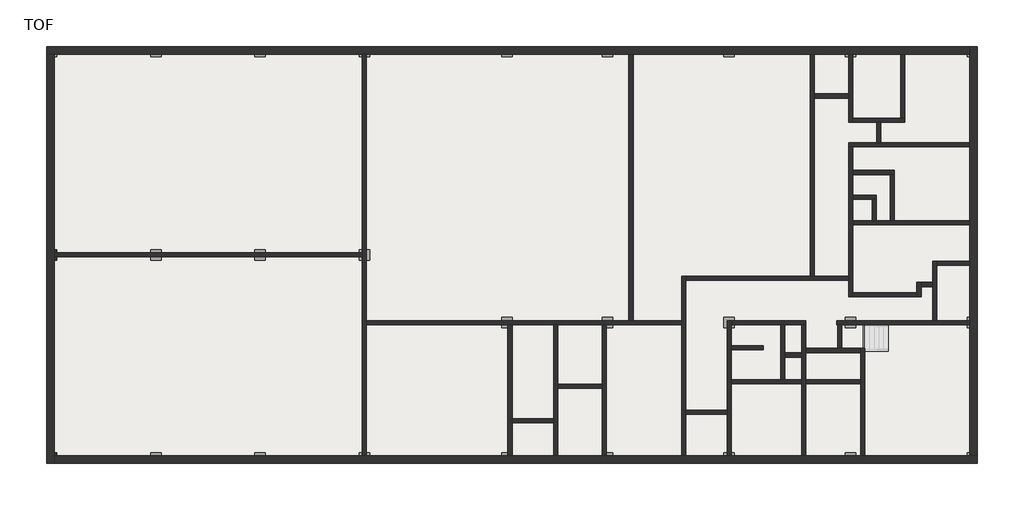
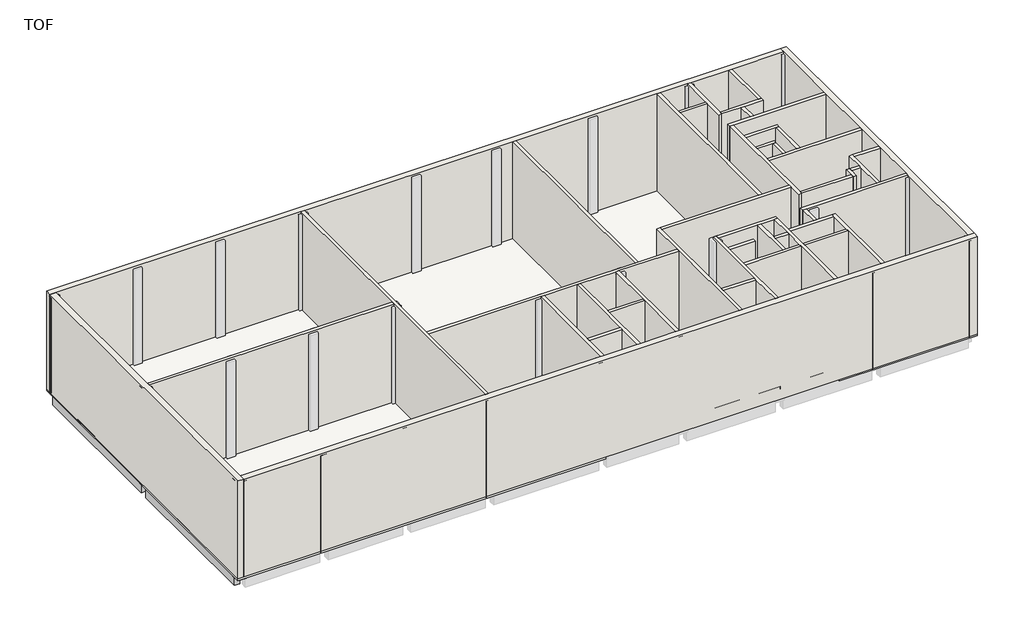
# One storey, part 1 of 2: 45 walls, 6 slabs, 2 beams, 2 columns.
# Revit data of these elements (continued)
# Element 13 (IfcWall, "H_WA_AMW_Brick Wall_Ext (0.5B_50_1.0B / Emulsion)") (continued)
#   Materials on its faces: "Default Wall"
# Element 14 (IfcWall, "H_WA_AMW_Brick Wall_Ext (0.5B_50_1.0B / Emulsion)")
#   Mark = "EW4"
#   Wall Loca = "EXT"
#   Wall Style Name = "Concrete Wall+Insulation+Gypsum Board"
#   Wall Base Material-2 = "Glass Wool (Fiberglass)"
#   Wall Base Material-3 = "Concrete Wall"
#   Wall Finish-Ex = "Acrylic Emulsion Paint on Fair Faced Concrete"
#   Top Offset = 0.000 mm
#   Base Offset = 0.000 mm
#   wall height = 7500.000 mm
#   Wall Style No = EW51-1
#   Phase Created = New Construction
#   Base Constraint = TOF
#   Top Constraint = TOC
#   Materials on its faces: "Default Wall"
# Element 15 (IfcWall, "H_WA_AMW_Block Wall_Int_T200 (Both Plaster_Emulsion)")
#   Mark = "W1"
#   Wall Loca = "INT"
#   Wall Style Name = "Block Wall"
#   Wall Ref. = ""
#   Wall Base Material-1 = "Concrete Block"
#   Wall Base Material-2 = ""
#   Wall Base Material-3 = ""
#   Wall Finish-Ex = ""
#   Top Offset = 0.000 mm
#   Base Offset = 0.000 mm
#   wall height = 7500.000 mm
#   Wall Style No = IW21
#   Phase Created = New Construction
#   Base Constraint = TOF
#   Top Constraint = TOC
#   Materials on its faces: "Default Wall"
# Element 16 (IfcWall, "H_WA_AMW_Block Wall_Int_T200 (Both Plaster_Emulsion)")
#   Mark = "W2"
#   Wall Loca = "INT"
#   Wall Style Name = "Block Wall"
#   Wall Ref. = ""
#   Wall Base Material-1 = "Concrete Block"
#   Wall Base Material-2 = ""
#   Wall Base Material-3 = ""
#   Wall Finish-Ex = ""
#   Top Offset = 0.000 mm
#   Base Offset = 0.000 mm
#   wall height = 7500.000 mm
#   Wall Style No = IW21
#   Phase Created = New Construction
#   Base Constraint = TOF
#   Top Constraint = TOC
#   Materials on its faces: "Default Wall"
# Element 17 (IfcWall, "H_WA_AMW_Block Wall_Int_T200 (Both Plaster_Emulsion)")
#   Mark = "W3"
#   Wall Loca = "INT"
#   Wall Style Name = "Block Wall"
#   Wall Ref. = ""
#   Wall Base Material-1 = "Concrete Block"
#   Wall Base Material-2 = ""
#   Wall Base Material-3 = ""
#   Wall Finish-Ex = ""
#   Top Offset = 0.000 mm
#   Base Offset = 0.000 mm
#   wall height = 7500.000 mm
#   Wall Style No = IW21
#   Phase Created = New Construction
#   Base Constraint = TOF
#   Top Constraint = TOC
#   Materials on its faces: "Default Wall"
# Element 18 (IfcWall, "H_WA_AMW_Block Wall_Int_T200 (Both Plaster_Emulsion)")
#   Mark = "W4"
#   Wall Loca = "INT"
#   Wall Style Name = "Block Wall"
#   Wall Ref. = ""
#   Wall Base Material-1 = "Concrete Block"
#   Wall Base Material-2 = ""
#   Wall Base Material-3 = ""
#   Wall Finish-Ex = ""
#   Top Offset = 0.000 mm
#   Base Offset = 0.000 mm
#   wall height = 7500.000 mm
#   Wall Style No = IW21
#   Phase Created = New Construction
#   Base Constraint = TOF
#   Top Constraint = TOC
#   Materials on its faces: "Default Wall"
# Element 19 (IfcWall, "H_WA_AMW_Block Wall_Int_T200 (Both Plaster_Emulsion)")
#   Mark = "W5"
#   Wall Loca = "INT"
#   Wall Style Name = "Block Wall"
#   Wall Ref. = ""
#   Wall Base Material-1 = "Concrete Block"
#   Wall Base Material-2 = ""
#   Wall Base Material-3 = ""
#   Wall Finish-Ex = ""
#   built-in parameter 1001111 = 1000.000 mm
#   Top Offset = 0.000 mm
#   Base Offset = 1000.000 mm
#   wall height = 6500.000 mm
#   Wall Style No = IW21
#   Phase Created = New Construction
#   Base Constraint = TOF
#   Top Constraint = TOC
#   Materials on its faces: "Default Wall"
# Element 20 (IfcWall, "H_WA_AMW_Block Wall_Int_T200 (Both Plaster_Emulsion)")
#   Mark = "W6"
#   Wall Loca = "INT"
#   Wall Style Name = "Block Wall"
#   Wall Ref. = ""
#   Wall Base Material-1 = "Concrete Block"
#   Wall Base Material-2 = ""
#   Wall Base Material-3 = ""
#   Wall Finish-Ex = ""
#   Top Offset = 0.000 mm
#   Base Offset = 0.000 mm
#   wall height = 7500.000 mm
#   Wall Style No = IW21
#   Phase Created = New Construction
#   Base Constraint = TOF
#   Top Constraint = TOC
#   Materials on its faces: "Default Wall"
# Element 21 (IfcWall, "H_WA_AMW_Block Wall_Int_T200 (Both Plaster_Emulsion)")
#   Mark = "W7"
#   Wall Loca = "INT"
#   Wall Style Name = "Block Wall"
#   Wall Ref. = ""
#   Wall Base Material-1 = "Concrete Block"
#   Wall Base Material-2 = ""
#   Wall Base Material-3 = ""
#   Wall Finish-Ex = ""
#   Top Offset = 0.000 mm
#   Base Offset = 0.000 mm
#   wall height = 7500.000 mm
#   Wall Style No = IW21
#   Phase Created = New Construction
#   Base Constraint = TOF
#   Top Constraint = TOC
#   Materials on its faces: "Default Wall"
# Element 22 (IfcWall, "H_WA_AMW_Block Wall_Int_T200 (Both Plaster_Emulsion)")
#   Mark = "W8"
#   Wall Loca = "INT"
#   Wall Style Name = "Block Wall"
#   Wall Ref. = ""
#   Wall Base Material-1 = "Concrete Block"
#   Wall Base Material-2 = ""
#   Wall Base Material-3 = ""
#   Wall Finish-Ex = ""
#   built-in parameter 1001111 = 1000.000 mm
#   Top Offset = 0.000 mm
#   Base Offset = 1000.000 mm
#   wall height = 6500.000 mm
#   Wall Style No = IW21
#   Phase Created = New Construction
#   Base Constraint = TOF
#   Top Constraint = TOC
#   Materials on its faces: "Default Wall"
# Element 23 (IfcWall, "H_WA_AMW_Block Wall_Int_T200 (Both Plaster_Emulsion)")
#   Mark = "W9"
#   Wall Loca = "INT"
#   Wall Style Name = "Block Wall"
#   Wall Ref. = ""
#   Wall Base Material-1 = "Concrete Block"
#   Wall Base Material-2 = ""
#   Wall Base Material-3 = ""
#   Wall Finish-Ex = ""
#   built-in parameter 1001111 = 1000.000 mm
#   Top Offset = 0.000 mm
#   Base Offset = 1000.000 mm
#   wall height = 6500.000 mm
#   Wall Style No = IW21
#   Phase Created = New Construction
#   Base Constraint = TOF
#   Top Constraint = TOC
#   Materials on its faces: "Default Wall"
# Element 24 (IfcWall, "H_WA_AMW_Block Wall_Int_T200 (Both Plaster_Emulsion)")
#   Mark = "W10"
#   Wall Loca = "INT"
#   Wall Style Name = "Block Wall"
#   Wall Ref. = ""
#   Wall Base Material-1 = "Concrete Block"
#   Wall Base Material-2 = ""
#   Wall Base Material-3 = ""
#   Wall Finish-Ex = ""
#   built-in parameter 1001111 = 1000.000 mm
#   Top Offset = 0.000 mm
#   Base Offset = 1000.000 mm
#   wall height = 6500.000 mm
#   Wall Style No = IW21
#   Phase Created = New Construction
#   Base Constraint = TOF
#   Top Constraint = TOC
#   Materials on its faces: "Default Wall"
# Element 25 (IfcWall, "H_WA_AMW_Block Wall_Int_T200 (Both Plaster_Emulsion)")
#   Mark = "W11"
#   Wall Loca = "INT"
#   Wall Style Name = "Block Wall"
#   Wall Ref. = ""
#   Wall Base Material-1 = "Concrete Block"
#   Wall Base Material-2 = ""
#   Wall Base Material-3 = ""
#   Wall Finish-Ex = ""
#   Top Offset = 0.000 mm
#   Base Offset = 0.000 mm
#   wall height = 7500.000 mm
#   Wall Style No = IW21
#   Phase Created = New Construction
#   Base Constraint = TOF
#   Top Constraint = TOC
#   Materials on its faces: "Default Wall"
# Element 26 (IfcWall, "H_WA_AMW_Block Wall_Int_T200 (Both Plaster_Emulsion)")
#   Mark = "W12"
#   Wall Loca = "INT"
#   Wall Style Name = "Block Wall"
#   Wall Ref. = ""
#   Wall Base Material-1 = "Concrete Block"
#   Wall Base Material-2 = ""
#   Wall Base Material-3 = ""
#   Wall Finish-Ex = ""
#   built-in parameter 1001111 = 1000.000 mm
#   Top Offset = 0.000 mm
#   Base Offset = 1000.000 mm
#   wall height = 6500.000 mm
#   Wall Style No = IW21
#   Phase Created = New Construction
#   Base Constraint = TOF
#   Top Constraint = TOC
#   Materials on its faces: "Default Wall"
# Element 27 (IfcWall, "H_WA_AMW_Block Wall_Int_T200 (Both Plaster_Emulsion)")
#   Mark = "W13"
#   Wall Loca = "INT"
#   Wall Style Name = "Block Wall"
#   Wall Ref. = ""
#   Wall Base Material-1 = "Concrete Block"
#   Wall Base Material-2 = ""
#   Wall Base Material-3 = ""
#   Wall Finish-Ex = ""
#   built-in parameter 1001111 = 1000.000 mm
#   Top Offset = 0.000 mm
#   Base Offset = 1000.000 mm
#   wall height = 6500.000 mm
#   Wall Style No = IW21
#   Phase Created = New Construction
#   Base Constraint = TOF
#   Top Constraint = TOC
#   Materials on its faces: "Default Wall"
# Element 28 (IfcWall, "H_WA_AMW_Block Wall_Int_T200 (Both Plaster_Emulsion)")
#   Mark = "W14"
#   Wall Loca = "INT"
#   Wall Style Name = "Block Wall"
#   Wall Ref. = ""
#   Wall Base Material-1 = "Concrete Block"
#   Wall Base Material-2 = ""
#   Wall Base Material-3 = ""
#   Wall Finish-Ex = ""
#   built-in parameter 1001111 = 1000.000 mm
#   Top Offset = 0.000 mm
#   Base Offset = 1000.000 mm
#   wall height = 6500.000 mm
#   Wall Style No = IW21
#   Phase Created = New Construction
#   Base Constraint = TOF
#   Top Constraint = TOC
#   Materials on its faces: "Default Wall"
# Element 29 (IfcWall, "H_WA_AMW_Block Wall_Int_T200 (Both Plaster_Emulsion)")
#   Mark = "W15"
#   Wall Loca = "INT"
#   Wall Style Name = "Block Wall"
#   Wall Ref. = ""
#   Wall Base Material-1 = "Concrete Block"
#   Wall Base Material-2 = ""
#   Wall Base Material-3 = ""
#   Wall Finish-Ex = ""
#   Top Offset = 0.000 mm
#   Base Offset = 0.000 mm
#   wall height = 7500.000 mm
#   Wall Style No = IW21
#   Phase Created = New Construction
#   Base Constraint = TOF
#   Top Constraint = TOC
#   Materials on its faces: "Default Wall"
# Element 30 (IfcWall, "H_WA_AMW_Block Wall_Int_T200 (Both Plaster_Emulsion)")
#   Mark = "W16"
#   Wall Loca = "INT"
#   Wall Style Name = "Block Wall"
#   Wall Ref. = ""
#   Wall Base Material-1 = "Concrete Block"
#   Wall Base Material-2 = ""
#   Wall Base Material-3 = ""
#   Wall Finish-Ex = ""
#   Top Offset = 0.000 mm
#   Base Offset = 0.000 mm
#   wall height = 7500.000 mm
#   Wall Style No = IW21
#   Phase Created = New Construction
#   Base Constraint = TOF
#   Top Constraint = TOC
#   Materials on its faces: "Default Wall"
# Element 31 (IfcWall, "H_WA_AMW_Block Wall_Int_T200 (Both Plaster_Emulsion)")
#   Mark = "W17"
#   Wall Loca = "INT"
#   Wall Style Name = "Block Wall"
#   Wall Ref. = ""
#   Wall Base Material-1 = "Concrete Block"
#   Wall Base Material-2 = ""
#   Wall Base Material-3 = ""
#   Wall Finish-Ex = ""
#   Top Offset = 0.000 mm
#   Base Offset = 0.000 mm
#   wall height = 7500.000 mm
#   Wall Style No = IW21
#   Phase Created = New Construction
#   Base Constraint = TOF
#   Top Constraint = TOC
#   Materials on its faces: "Default Wall"
# Element 32 (IfcWall, "H_WA_AMW_Block Wall_Int_T200 (Both Plaster_Emulsion)")
#   Mark = "W18"
#   Wall Loca = "INT"
#   Wall Style Name = "Block Wall"
#   Wall Ref. = ""
#   Wall Base Material-1 = "Concrete Block"
#   Wall Base Material-2 = ""
#   Wall Base Material-3 = ""
#   Wall Finish-Ex = ""
#   Top Offset = 0.000 mm
#   Base Offset = 0.000 mm
#   wall height = 7500.000 mm
#   Wall Style No = IW21
#   Phase Created = New Construction
#   Base Constraint = TOF
#   Top Constraint = TOC
#   Materials on its faces: "Default Wall"
# Element 33 (IfcWall, "H_WA_AMW_Block Wall_Int_T200 (Both Plaster_Emulsion)")
#   Mark = "W19"
#   Wall Loca = "INT"
#   Wall Style Name = "Block Wall"
#   Wall Ref. = ""
#   Wall Base Material-1 = "Concrete Block"
#   Wall Base Material-2 = ""
#   Wall Base Material-3 = ""
#   Wall Finish-Ex = ""
#   Top Offset = 0.000 mm
#   Base Offset = 0.000 mm
#   wall height = 7500.000 mm
#   Wall Style No = IW21
#   Phase Created = New Construction
#   Base Constraint = TOF
#   Top Constraint = TOC
#   Materials on its faces: "Default Wall"
# Element 34 (IfcWall, "H_WA_AMW_Block Wall_Int_T200 (Both Plaster_Emulsion)")
#   Mark = "W20"
#   Wall Loca = "INT"
#   Wall Style Name = "Block Wall"
#   Wall Ref. = ""
#   Wall Base Material-1 = "Concrete Block"
#   Wall Base Material-2 = ""
#   Wall Base Material-3 = ""
#   Wall Finish-Ex = ""
#   Top Offset = 0.000 mm
#   Base Offset = 0.000 mm
#   wall height = 7500.000 mm
#   Wall Style No = IW21
#   Phase Created = New Construction
#   Base Constraint = TOF
#   Top Constraint = TOC
#   Materials on its faces: "Default Wall"
# Element 35 (IfcWall, "H_WA_AMW_Block Wall_Int_T200 (Both Plaster_Emulsion)")
#   Mark = "W21"
#   Wall Loca = "INT"
#   Wall Style Name = "Block Wall"
#   Wall Ref. = ""
#   Wall Base Material-1 = "Concrete Block"
#   Wall Base Material-2 = ""
#   Wall Base Material-3 = ""
#   Wall Finish-Ex = ""
#   Top Offset = 0.000 mm
#   Base Offset = 0.000 mm
#   wall height = 7500.000 mm
#   Wall Style No = IW21
#   Phase Created = New Construction
#   Base Constraint = TOF
#   Top Constraint = TOC
#   Materials on its faces: "Default Wall"
# Element 36 (IfcWall, "H_WA_AMW_Block Wall_Int_T200 (Both Plaster_Emulsion)")
#   Mark = "W22"
#   Wall Loca = "INT"
#   Wall Style Name = "Block Wall"
#   Wall Ref. = ""
#   Wall Base Material-1 = "Concrete Block"
#   Wall Base Material-2 = ""
#   Wall Base Material-3 = ""
#   Wall Finish-Ex = ""
#   Top Offset = 0.000 mm
#   Base Offset = 0.000 mm
#   wall height = 7500.000 mm
#   Wall Style No = IW21
#   Phase Created = New Construction
#   Base Constraint = TOF
#   Top Constraint = TOC
#   Materials on its faces: "Default Wall"
# Element 37 (IfcWall, "H_WA_AMW_Block Wall_Int_T200 (Both Plaster_Emulsion)")
#   Mark = "W23"
#   Wall Loca = "INT"
#   Wall Style Name = "Block Wall"
#   Wall Ref. = ""
#   Wall Base Material-1 = "Concrete Block"
#   Wall Base Material-2 = ""
#   Wall Base Material-3 = ""
#   Wall Finish-Ex = ""
#   Top Offset = 0.000 mm
#   Base Offset = 0.000 mm
#   wall height = 7500.000 mm
#   Wall Style No = IW21
#   Phase Created = New Construction
#   Base Constraint = TOF
#   Top Constraint = TOC
#   Materials on its faces: "Default Wall"
# Element 38 (IfcWall, "H_WA_AMW_Block Wall_Int_T200 (Both Plaster_Emulsion)")
#   Mark = "W24"
#   Wall Loca = "INT"
#   Wall Style Name = "Block Wall"
#   Wall Ref. = ""
#   Wall Base Material-1 = "Concrete Block"
#   Wall Base Material-2 = ""
#   Wall Base Material-3 = ""
#   Wall Finish-Ex = ""
#   Top Offset = 0.000 mm
#   Base Offset = 0.000 mm
#   wall height = 7500.000 mm
#   Wall Style No = IW21
#   Phase Created = New Construction
#   Base Constraint = TOF
#   Top Constraint = TOC
#   Materials on its faces: "Default Wall"
# Element 39 (IfcWall, "H_WA_AMW_Block Wall_Int_T200 (Both Plaster_Emulsion)")
#   Mark = "W25"
#   Wall Loca = "INT"
#   Wall Style Name = "Block Wall"
#   Wall Ref. = ""
#   Wall Base Material-1 = "Concrete Block"
#   Wall Base Material-2 = ""
#   Wall Base Material-3 = ""
#   Wall Finish-Ex = ""
#   built-in parameter 1001111 = 1000.000 mm
#   Top Offset = 0.000 mm
#   Base Offset = 1000.000 mm
#   wall height = 6500.000 mm
#   Wall Style No = IW21
#   Phase Created = New Construction
#   Base Constraint = TOF
#   Top Constraint = TOC
#   Materials on its faces: "Default Wall"
# Element 40 (IfcWall, "H_WA_AMW_Block Wall_Int_T200 (Both Plaster_Emulsion)")
#   Mark = "W26"
#   Wall Loca = "INT"
#   Wall Style Name = "Block Wall"
#   Wall Ref. = ""
#   Wall Base Material-1 = "Concrete Block"
#   Wall Base Material-2 = ""
#   Wall Base Material-3 = ""
#   Wall Finish-Ex = ""
#   built-in parameter 1001111 = 1000.000 mm
#   Top Offset = 0.000 mm
#   Base Offset = 1000.000 mm
#   wall height = 6500.000 mm
#   Wall Style No = IW21
#   Phase Created = New Construction
#   Base Constraint = TOF
#   Top Constraint = TOC
#   Materials on its faces: "Default Wall"
# Element 41 (IfcWall, "H_WA_AMW_Block Wall_Int_T200 (Both Plaster_Emulsion)")
#   Mark = "W27"
#   Wall Loca = "INT"
#   Wall Style Name = "Block Wall"
#   Wall Ref. = ""
#   Wall Base Material-1 = "Concrete Block"
#   Wall Base Material-2 = ""
#   Wall Base Material-3 = ""
#   Wall Finish-Ex = ""
#   Top Offset = 0.000 mm
#   Base Offset = 0.000 mm
#   wall height = 7500.000 mm
#   Wall Style No = IW21
#   Phase Created = New Construction
#   Base Constraint = TOF
#   Top Constraint = TOC
#   Materials on its faces: "Default Wall"
# Element 42 (IfcWall, "H_WA_AMW_Block Wall_Int_T200 (Both Plaster_Emulsion)")
#   Mark = "W28"
#   Wall Loca = "INT"
#   Wall Style Name = "Block Wall"
#   Wall Ref. = ""
#   Wall Base Material-1 = "Concrete Block"
#   Wall Base Material-2 = ""
#   Wall Base Material-3 = ""
#   Wall Finish-Ex = ""
#   built-in parameter 1001111 = 1000.000 mm
#   Top Offset = 0.000 mm
#   Base Offset = 1000.000 mm
#   wall height = 6500.000 mm
#   Wall Style No = IW21
#   Phase Created = New Construction
#   Base Constraint = TOF
#   Top Constraint = TOC
#   Materials on its faces: "Default Wall"
# Element 43 (IfcWall, "H_WA_AMW_Block Wall_Int_T200 (Both Plaster_Emulsion)")
#   Mark = "W29"
#   Wall Loca = "INT"
#   Wall Style Name = "Block Wall"
#   Wall Ref. = ""
#   Wall Base Material-1 = "Concrete Block"
#   Wall Base Material-2 = ""
#   Wall Base Material-3 = ""
#   Wall Finish-Ex = ""
#   built-in parameter 1001111 = 1000.000 mm
#   Top Offset = 0.000 mm
#   Base Offset = 1000.000 mm
#   wall height = 6500.000 mm
#   Wall Style No = IW21
#   Phase Created = New Construction
#   Base Constraint = TOF
#   Top Constraint = TOC
#   Materials on its faces: "Default Wall"
# Element 44 (IfcWall, "H_WA_AMW_Block Wall_Int_T200 (Both Plaster_Emulsion)")
#   Mark = "W30"
#   Wall Loca = "INT"
#   Wall Style Name = "Block Wall"
#   Wall Ref. = ""
#   Wall Base Material-1 = "Concrete Block"
#   Wall Base Material-2 = ""
#   Wall Base Material-3 = ""
#   Wall Finish-Ex = ""
#   built-in parameter 1001111 = 1000.000 mm
#   Top Offset = 0.000 mm
#   Base Offset = 1000.000 mm
#   wall height = 6500.000 mm
#   Wall Style No = IW21
#   Phase Created = New Construction
#   Base Constraint = TOF
#   Top Constraint = TOC
#   Materials on its faces: "Default Wall"
# Element 45 (IfcWall, "H_WA_AMW_Block Wall_Int_T200 (Both Plaster_Emulsion)")
#   Mark = "W31"
#   Wall Loca = "INT"
#   Wall Style Name = "Block Wall"
#   Wall Ref. = ""
#   Wall Base Material-1 = "Concrete Block"
#   Wall Base Material-2 = ""
#   Wall Base Material-3 = ""
#   Wall Finish-Ex = ""
#   built-in parameter 1001111 = 1000.000 mm
#   Top Offset = 0.000 mm
#   Base Offset = 1000.000 mm
#   wall height = 6500.000 mm
#   Wall Style No = IW21
#   Phase Created = New Construction
#   Base Constraint = TOF
#   Top Constraint = TOC
#   Materials on its faces: "Default Wall"
# Element 46 (IfcWall, "H_WA_AMW_Block Wall_Int_T200 (Both Plaster_Emulsion)")
#   Mark = "W32"
#   Wall Loca = "INT"
#   Wall Style Name = "Block Wall"
#   Wall Ref. = ""
#   Wall Base Material-1 = "Concrete Block"
#   Wall Base Material-2 = ""
#   Wall Base Material-3 = ""
#   Wall Finish-Ex = ""
#   built-in parameter 1001111 = 1000.000 mm
#   Top Offset = 0.000 mm
#   Base Offset = 1000.000 mm
#   wall height = 6500.000 mm
#   Wall Style No = IW21
#   Phase Created = New Construction
#   Base Constraint = TOF
#   Top Constraint = TOC
#   Materials on its faces: "Default Wall"
# Element 47 (IfcWall, "H_WA_AMW_Block Wall_Int_T200 (Both Plaster_Emulsion)")
#   Mark = "W33"
#   Wall Loca = "INT"
#   Wall Style Name = "Block Wall"
#   Wall Ref. = ""
#   Wall Base Material-1 = "Concrete Block"
#   Wall Base Material-2 = ""
#   Wall Base Material-3 = ""
#   Wall Finish-Ex = ""
#   built-in parameter 1001111 = 1000.000 mm
#   Top Offset = 0.000 mm
#   Base Offset = 1000.000 mm
#   wall height = 6500.000 mm
#   Wall Style No = IW21
#   Phase Created = New Construction
#   Base Constraint = TOF
#   Top Constraint = TOC
#   Materials on its faces: "Default Wall"
# Element 48 (IfcWall, "H_WA_AMW_Block Wall_Int_T200 (Both Plaster_Emulsion)")
#   Mark = "W34"
#   Wall Loca = "INT"
#   Wall Style Name = "Block Wall"
#   Wall Ref. = ""
#   Wall Base Material-1 = "Concrete Block"
#   Wall Base Material-2 = ""
#   Wall Base Material-3 = ""
#   Wall Finish-Ex = ""
#   built-in parameter 1001111 = 1000.000 mm
#   Top Offset = 0.000 mm
#   Base Offset = 1000.000 mm
#   wall height = 6500.000 mm
#   Wall Style No = IW21
#   Phase Created = New Construction
#   Base Constraint = TOF
#   Top Constraint = TOC
#   Materials on its faces: "Default Wall"
# Element 49 (IfcWall, "H_WA_AMW_Block Wall_Int_T200 (Both Plaster_Emulsion)")
#   Mark = "W35"
#   Wall Loca = "INT"
#   Wall Style Name = "Block Wall"
#   Wall Ref. = ""
#   Wall Base Material-1 = "Concrete Block"
#   Wall Base Material-2 = ""
#   Wall Base Material-3 = ""
#   Wall Finish-Ex = ""
#   built-in parameter 1001111 = 1000.000 mm
#   Top Offset = 0.000 mm
#   Base Offset = 1000.000 mm
#   wall height = 6500.000 mm
#   Wall Style No = IW21
#   Phase Created = New Construction
#   Base Constraint = TOF
#   Top Constraint = TOC
#   Materials on its faces: "Default Wall"
# Element 50 (IfcWall, "H_WA_AMW_Block Wall_Int_T200 (Both Plaster_Emulsion)")
#   Mark = "W36"
#   Wall Loca = "INT"
#   Wall Style Name = "Block Wall"
#   Wall Ref. = ""
#   Wall Base Material-1 = "Concrete Block"
#   Wall Base Material-2 = ""
#   Wall Base Material-3 = ""
#   Wall Finish-Ex = ""
#   built-in parameter 1001111 = 1000.000 mm
#   Top Offset = 0.000 mm
#   Base Offset = 1000.000 mm
#   wall height = 6500.000 mm
#   Wall Style No = IW21
#   Phase Created = New Construction
#   Base Constraint = TOF
#   Top Constraint = TOC
#   Materials on its faces: "Default Wall"
# Element 51 (IfcWall, "H_WA_AMW_Block Wall_Int_T200 (Both Plaster_Emulsion)")
#   Mark = "W37"
#   Wall Loca = "INT"
#   Wall Style Name = "Block Wall"
#   Wall Ref. = ""
#   Wall Base Material-1 = "Concrete Block"
#   Wall Base Material-2 = ""
#   Wall Base Material-3 = ""
#   Wall Finish-Ex = ""
#   built-in parameter 1001111 = 1000.000 mm
#   Top Offset = 0.000 mm
#   Base Offset = 1000.000 mm
#   wall height = 6500.000 mm
#   Wall Style No = IW21
#   Phase Created = New Construction
#   Base Constraint = TOF
#   Top Constraint = TOC
#   Materials on its faces: "Default Wall"
# Element 52 (IfcWall, "H_WA_AMW_Block Wall_Int_T200 (Both Plaster_Emulsion)")
#   Mark = "W38"
#   Wall Loca = "INT"
#   Wall Style Name = "Block Wall"
#   Wall Ref. = ""
#   Wall Base Material-1 = "Concrete Block"
#   Wall Base Material-2 = ""
#   Wall Base Material-3 = ""
#   Wall Finish-Ex = ""
#   built-in parameter 1001111 = 1000.000 mm
#   Top Offset = 0.000 mm
#   Base Offset = 1000.000 mm
#   wall height = 6500.000 mm
#   Wall Style No = IW21
#   Phase Created = New Construction
#   Base Constraint = TOF
#   Top Constraint = TOC
#   Materials on its faces: "Default Wall"
# Element 53 (IfcWall, "H_WA_AMW_Block Wall_Int_T200 (Both Plaster_Emulsion)")
#   Mark = "W39"
#   Wall Loca = "INT"
#   Wall Style Name = "Block Wall"
#   Wall Ref. = ""
#   Wall Base Material-1 = "Concrete Block"
#   Wall Base Material-2 = ""
#   Wall Base Material-3 = ""
#   Wall Finish-Ex = ""
#   built-in parameter 1001111 = 1000.000 mm
#   Top Offset = 0.000 mm
#   Base Offset = 1000.000 mm
#   wall height = 6500.000 mm
#   Wall Style No = IW21
#   Phase Created = New Construction
#   Base Constraint = TOF
#   Top Constraint = TOC
#   Materials on its faces: "Default Wall"
# Element 54 (IfcWall, "H_WA_AMW_Block Wall_Int_T200 (Both Plaster_Emulsion)")
#   Mark = "W40"
#   Wall Loca = "INT"
#   Wall Style Name = "Block Wall"
#   Wall Ref. = ""
#   Wall Base Material-1 = "Concrete Block"
#   Wall Base Material-2 = ""
#   Wall Base Material-3 = ""
#   Wall Finish-Ex = ""
#   built-in parameter 1001111 = 1000.000 mm
#   Top Offset = 0.000 mm
#   Base Offset = 1000.000 mm
#   wall height = 6500.000 mm
#   Wall Style No = IW21
#   Phase Created = New Construction
#   Base Constraint = TOF
#   Top Constraint = TOC
#   Materials on its faces: "Default Wall"
# Element 55 (IfcWall, "H_WA_AMW_Block Wall_Int_T200 (Both Plaster_Emulsion)")
#   Mark = "W41"
#   Wall Loca = "INT"
#   Wall Style Name = "Block Wall"
#   Wall Ref. = ""
#   Wall Base Material-1 = "Concrete Block"
#   Wall Base Material-2 = ""
#   Wall Base Material-3 = ""
#   Wall Finish-Ex = ""
#   Top Offset = 0.000 mm
#   Base Offset = 0.000 mm
#   wall height = 7500.000 mm
#   Wall Style No = IW21
#   Phase Created = New Construction
#   Base Constraint = TOF
#   Top Constraint = TOC
#   Materials on its faces: "Default Wall"
# Materials
#   "Default Floor": class "Miscellaneous", colour RGB 80 80 80, transparency 0
#   "Default Wall": class "Miscellaneous", colour RGB 80 80 80, transparency 0
